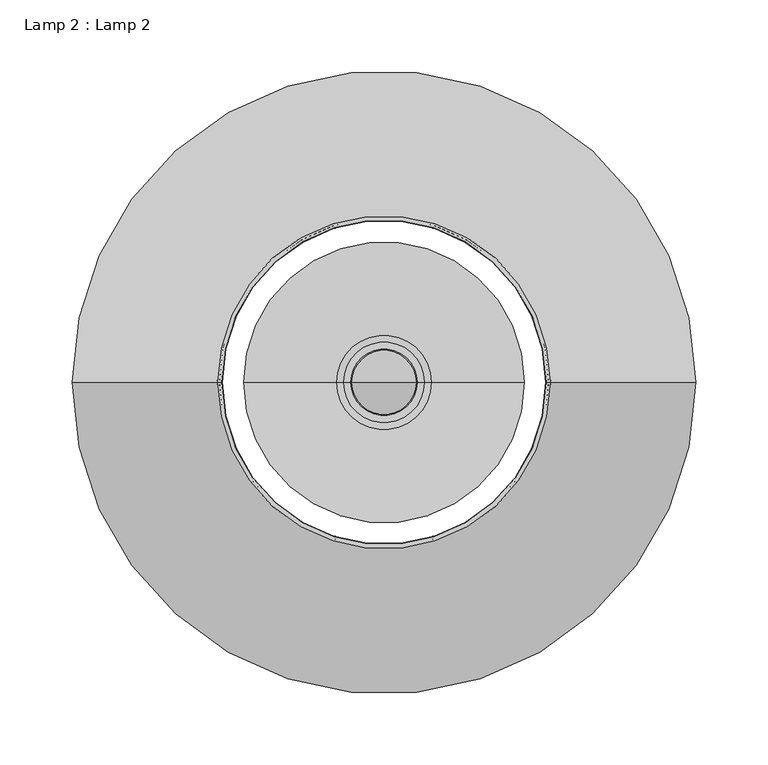
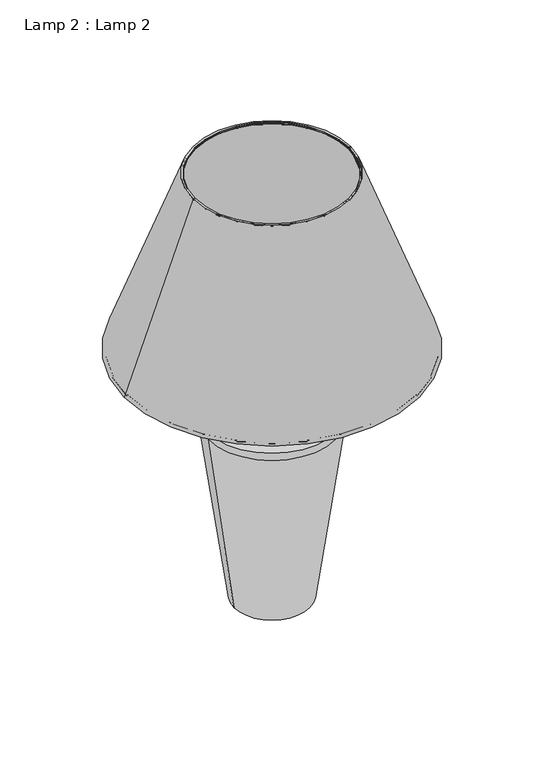
"""IFC4 building model written with IfcOpenShell, lengths in millimetres: furniture geometry, Lamp 2 : Lamp 2."""

import ifcopenshell
import ifcopenshell.guid

model = None  # the IFC model being written
_history = None  # IfcOwnerHistory: only IFC2X3 demands one
_inside = {}  # id of a spatial element -> (the spatial element, [elements in it])
_under = {}  # id of a project, library or spatial element -> (it, [spatial elements below it])
_declared = {}  # id of a project -> (the project, [libraries it declares])
_typed = {}  # id of a type object -> (the type object, [elements of that type])
_made_of = {}  # id of a material, layer set ... -> (it, [elements and type objects made of it])


def new_model(schema):
    """Start an empty IFC model of exactly this schema.

    Asked for "IFC4X3", IfcOpenShell would pick the latest addendum, in which some entities
    have other attributes; the version numbers below select the first issue.
    IFC2X3 requires an IfcOwnerHistory on every rooted entity: one is made here for all.
    """
    global model, _history
    if schema == "IFC4X3":
        model = ifcopenshell.file(schema_version=(4, 3, 0, 0))
    else:
        model = ifcopenshell.file(schema=schema)
    _inside.clear()
    _under.clear()
    _declared.clear()
    _typed.clear()
    _made_of.clear()
    _history = None
    if model.schema == "IFC2X3":
        org = make("IfcOrganization", Name="unknown")
        user = make(
            "IfcPersonAndOrganization",
            ThePerson=make("IfcPerson", FamilyName="unknown"),
            TheOrganization=org,
        )
        app = make(
            "IfcApplication",
            ApplicationDeveloper=org,
            Version="unknown",
            ApplicationFullName="unknown",
            ApplicationIdentifier="unknown",
        )
        _history = make(
            "IfcOwnerHistory",
            OwningUser=user,
            OwningApplication=app,
            ChangeAction="ADDED",
            CreationDate=0,
        )
    return model


def make(cls, **values):
    """One entity of the class cls with the attributes given. An attribute that is None is left unset."""
    return model.create_entity(
        cls, **{name: value for name, value in values.items() if value is not None}
    )


def rooted(cls, **values):
    """An entity with a GlobalId (a new one), such as an element, a storey or a relation."""
    return make(cls, GlobalId=ifcopenshell.guid.new(), OwnerHistory=_history, **values)


def si_unit(unit_type, name, prefix=None):
    """IfcSIUnit, for example si_unit("LENGTHUNIT", "METRE", prefix="MILLI")."""
    return make("IfcSIUnit", UnitType=unit_type, Prefix=prefix, Name=name)


def assignment(units):
    """IfcUnitAssignment: the units of a project."""
    return None if units is None else make("IfcUnitAssignment", Units=units)


def point(xyz):
    """IfcCartesianPoint."""
    return None if xyz is None else make("IfcCartesianPoint", Coordinates=xyz)


def direction(xyz):
    """IfcDirection."""
    return None if xyz is None else make("IfcDirection", DirectionRatios=xyz)


def frame(location, z_axis=None, x_axis=None):
    """IfcAxis2Placement3D, a coordinate frame: its origin and axes. An axis left out is left unset."""
    return make(
        "IfcAxis2Placement3D",
        Location=point(location),
        Axis=direction(z_axis),
        RefDirection=direction(x_axis),
    )


def origin():
    """The frame at (0, 0, 0) with its axes left unset."""
    return frame((0.0, 0.0, 0.0))


def place(relative_to, where):
    """IfcLocalPlacement: puts the frame where relative to a parent placement (None: the world)."""
    return make(
        "IfcLocalPlacement", PlacementRelTo=relative_to, RelativePlacement=where
    )


def context(
    kind, dimensions, precision=None, world=None, true_north=None, identifier=None
):
    """IfcGeometricRepresentationContext, for example the 3D "Model" context."""
    return make(
        "IfcGeometricRepresentationContext",
        ContextIdentifier=identifier,
        ContextType=kind,
        CoordinateSpaceDimension=dimensions,
        Precision=precision,
        WorldCoordinateSystem=world,
        TrueNorth=true_north,
    )


def project(units=None, contexts=None):
    """IfcProject with its units and contexts."""
    return rooted(
        "IfcProject",
        Name="project",
        RepresentationContexts=contexts,
        UnitsInContext=assignment(units),
    )


def spatial(cls, under=None, at=None, **own):
    """A site, building, storey or space (cls), placed at a placement, below another one or the project."""
    s = rooted(cls, ObjectPlacement=at, **own)
    if under is not None:
        _under.setdefault(under.id(), (under, []))[1].append(s)
    return s


def polyline(points):
    """IfcPolyline through the points."""
    return make("IfcPolyline", Points=[point(p) for p in points])


def circle_curve(where, radius):
    """IfcCircle in the frame where."""
    return make("IfcCircle", Position=where, Radius=radius)


def ellipse_curve(where, semi_axis1, semi_axis2):
    """IfcEllipse in the frame where."""
    return make(
        "IfcEllipse", Position=where, SemiAxis1=semi_axis1, SemiAxis2=semi_axis2
    )


def trimmed(basis, trim1, trim2, sense, master):
    """IfcTrimmedCurve: the piece of a basis curve between two trims."""
    return make(
        "IfcTrimmedCurve",
        BasisCurve=basis,
        Trim1=trim1,
        Trim2=trim2,
        SenseAgreement=sense,
        MasterRepresentation=master,
    )


def shape(context_of_items, identifier, shape_type, items):
    """IfcShapeRepresentation: the items that make up one representation, for example the "Body"."""
    return make(
        "IfcShapeRepresentation",
        ContextOfItems=context_of_items,
        RepresentationIdentifier=identifier,
        RepresentationType=shape_type,
        Items=items,
    )


def source(mapping_origin, context_of_items, identifier, shape_type, items):
    """IfcRepresentationMap: a shape defined once, which mapped items show again and again."""
    return make(
        "IfcRepresentationMap",
        MappingOrigin=mapping_origin,
        MappedRepresentation=shape(context_of_items, identifier, shape_type, items),
    )


def transform(
    local_origin,
    x_axis=None,
    y_axis=None,
    z_axis=None,
    scale=None,
    scale2=None,
    scale3=None,
    uniform=True,
):
    """IfcCartesianTransformationOperator3D, or its non-uniform kind. x_axis, y_axis, z_axis: its Axis1, 2, 3."""
    if uniform:
        return make(
            "IfcCartesianTransformationOperator3D",
            Axis1=direction(x_axis),
            Axis2=direction(y_axis),
            LocalOrigin=point(local_origin),
            Scale=scale,
            Axis3=direction(z_axis),
        )
    return make(
        "IfcCartesianTransformationOperator3DnonUniform",
        Axis1=direction(x_axis),
        Axis2=direction(y_axis),
        LocalOrigin=point(local_origin),
        Scale=scale,
        Axis3=direction(z_axis),
        Scale2=scale2,
        Scale3=scale3,
    )


def mapped(mapping_source, mapping_target):
    """IfcMappedItem: shows the shape of a source again, moved by a transform."""
    return make(
        "IfcMappedItem", MappingSource=mapping_source, MappingTarget=mapping_target
    )


def made_of(thing, what):
    """Note that an element or type object is made of a material, layer set ...; save() writes the relation."""
    if what is not None:
        _made_of.setdefault(what.id(), (what, []))[1].append(thing)
    return thing


def element(
    cls,
    number,
    at=None,
    inside=None,
    cuts=None,
    type_object=None,
    material=None,
    context=None,
    identifier="Body",
    shape_type=None,
    held_by="IfcProductDefinitionShape",
    body=None,
    shapes=None,
    **own,
):
    """One element of the class cls, such as IfcWall. Its Tag is "e" and its number.

    at: its placement. inside: the storey or other place that contains it. cuts: it is an
    opening in that element (IfcRelVoidsElement). A single representation is given by context,
    identifier, shape_type and body (its items); several are given by shapes. held_by: the class
    of the entity that holds the representations. save() writes the other relations.
    """
    e = rooted(cls, Tag="e%d" % number, ObjectPlacement=at, **own)
    if body is not None:
        shapes = [shape(context, identifier, shape_type, body)]
    if shapes is not None:
        e.Representation = make(held_by, Representations=shapes)
    if inside is not None:
        _inside.setdefault(inside.id(), (inside, []))[1].append(e)
    if cuts is not None:
        rooted(
            "IfcRelVoidsElement", RelatingBuildingElement=cuts, RelatedOpeningElement=e
        )
    if type_object is not None:
        _typed.setdefault(type_object.id(), (type_object, []))[1].append(e)
    return made_of(e, material)


def aggregate(whole, parts):
    """IfcRelAggregates: a whole, such as a stair, and the parts it consists of."""
    return rooted("IfcRelAggregates", RelatingObject=whole, RelatedObjects=parts)


def save(model, path):
    """Write the relations noted so far, then the file.

    IfcRelAggregates (storeys below a building ...), IfcRelContainedInSpatialStructure (elements
    in a storey), IfcRelDefinesByType, IfcRelAssociatesMaterial and IfcRelDeclares: one each for
    every whole, place, type object, material and project.
    """
    for whole, parts in _under.values():
        aggregate(whole, parts)
    for where, things in _inside.values():
        rooted(
            "IfcRelContainedInSpatialStructure",
            RelatedElements=things,
            RelatingStructure=where,
        )
    for kind, things in _typed.values():
        rooted("IfcRelDefinesByType", RelatedObjects=things, RelatingType=kind)
    for what, things in _made_of.values():
        rooted("IfcRelAssociatesMaterial", RelatedObjects=things, RelatingMaterial=what)
    for by, libraries in _declared.values():
        rooted("IfcRelDeclares", RelatingContext=by, RelatedDefinitions=libraries)
    model.write(path)


def plane_surface(at):
    """IfcPlane: the flat surface through the origin of the frame at, square to its z axis."""
    return make("IfcPlane", Position=at)


def cylinder_surface(at, radius):
    """IfcCylindricalSurface: all points at the distance radius from the z axis of the frame at."""
    return make("IfcCylindricalSurface", Position=at, Radius=radius)


def revolved_surface(curve, axis_point, axis_direction):
    """IfcSurfaceOfRevolution: the curve turned about the line through axis_point along axis_direction."""
    return make(
        "IfcSurfaceOfRevolution",
        SweptCurve=make("IfcArbitraryOpenProfileDef", ProfileType="CURVE", Curve=curve),
        AxisPosition=make("IfcAxis1Placement", Location=point(axis_point), Axis=direction(axis_direction)),
    )


def spline_curve(degree, points, multiplicities, knots, weights=None):
    """IfcBSplineCurveWithKnots; with weights, IfcRationalBSplineCurveWithKnots."""
    own = dict(
        Degree=degree,
        ControlPointsList=[point(p) for p in points],
        CurveForm="UNSPECIFIED",
        ClosedCurve=False,
        SelfIntersect=False,
        KnotMultiplicities=multiplicities,
        Knots=knots,
        KnotSpec="UNSPECIFIED",
    )
    if weights is None:
        return make("IfcBSplineCurveWithKnots", **own)
    return make("IfcRationalBSplineCurveWithKnots", WeightsData=weights, **own)


def advanced_brep(points, edges, surfaces, faces):
    """IfcAdvancedBrep: a solid bounded by faces that lie on surfaces and meet in shared edges.

    An edge is (start, end): straight between two places in points (the first is 0);
    or (start, end, curve); or (start, end, curve, False) where it runs against its curve.
    A face is (place in surfaces, loops), or (place, loops, False) where it looks against
    its surface's normal. A loop lists edges by number (the first is 1), with a minus sign
    where the edge is run from its end to its start. The first loop is the outer one.
    """
    corners = [point(p) for p in points]
    vertices = [make("IfcVertexPoint", VertexGeometry=c) for c in corners]
    made = []
    for start, end, *more in edges:
        made.append(
            make(
                "IfcEdgeCurve",
                EdgeStart=vertices[start],
                EdgeEnd=vertices[end],
                EdgeGeometry=more[0] if more else make("IfcPolyline", Points=[corners[start], corners[end]]),
                SameSense=more[1] if len(more) > 1 else True,
            )
        )
    hull = []
    for where, loops, *sense in faces:
        bounds = []
        for j, loop in enumerate(loops):
            ring = [make("IfcOrientedEdge", EdgeElement=made[abs(k) - 1], Orientation=k > 0) for k in loop]
            bounds.append(
                make(
                    "IfcFaceOuterBound" if j == 0 else "IfcFaceBound",
                    Bound=make("IfcEdgeLoop", EdgeList=ring),
                    Orientation=True,
                )
            )
        hull.append(make("IfcAdvancedFace", Bounds=bounds, FaceSurface=surfaces[where], SameSense=sense[0] if sense else True))
    return make("IfcAdvancedBrep", Outer=make("IfcClosedShell", CfsFaces=hull))


def lamp_2_lamp_2_ee5345a8(model_context):
    return source(origin(), model_context, "Body", "AdvancedBrep", [
        advanced_brep(
        [(-5.625, 0.0049096, 408.6874636), (5.625, 0.0049096, 408.6874636), (5.625, 0.0049096, 396.7479044), (-5.625, 0.0049096, 396.7479044), (0.0, 0.0049096, 452.3091199), (0.0, 0.0049096, 396.7479044)],
        [
            (0, 1, circle_curve(frame((0.0, 0.0049096, 408.6874636), z_axis=(0.0, 0.0, -1.0), x_axis=(1.0, 0.0, 0.0)), 5.625)),
            (1, 2),
            (2, 3, circle_curve(frame((0.0, 0.0049096, 396.7479044), z_axis=(0.0, 0.0, 1.0), x_axis=(1.0, 0.0, 0.0)), 5.625)),
            (3, 0),
            (1, 0, circle_curve(frame((0.0, 0.0049096, 408.6874636), z_axis=(0.0, 0.0, -1.0), x_axis=(1.0, 0.0, 0.0)), 5.625)),
            (3, 2, circle_curve(frame((0.0, 0.0049096, 396.7479044), z_axis=(0.0, 0.0, 1.0), x_axis=(1.0, 0.0, 0.0)), 5.625)),
            (4, 1, circle_curve(frame((0.0, 0.0049096, 430.1356207), z_axis=(0.0, 1.0, 0.0), x_axis=(1.0, 0.0, 0.0)), 22.1734992)),
            (0, 4, circle_curve(frame((0.0, 0.0049096, 430.1356207), z_axis=(0.0, 1.0, 0.0), x_axis=(-1.0, 0.0, 0.0)), 22.1734992)),
            (2, 5),
            (5, 3),
        ],
        [
            cylinder_surface(frame((0.0, 0.0049096, 452.3091199), z_axis=(0.0, 0.0, 1.0), x_axis=(1.0, 0.0, 0.0)), 5.625),
            revolved_surface(trimmed(ellipse_curve(frame((0.0, 0.0049096, 430.1356207), z_axis=(0.0, -1.0, 0.0), x_axis=(1.0, 0.0, 0.0)), 22.1734992, 22.1734992), [point((5.625, 0.0049096, 408.6874636))], [point((0.0, 0.0049096, 452.3091199))], True, "CARTESIAN"), (0.0, 0.0049096, 452.3091199), (0.0, 0.0, 1.0)),
            plane_surface(frame((0.0, 0.0049096, 396.7479044), z_axis=(0.0, 0.0, -1.0), x_axis=(1.0, 0.0, 0.0))),
        ],
        [
            (0, [[1, 2, 3, 4]]),
            (0, [[5, -4, 6, -2]]),
            (1, [[7, -1, 8]]),
            (1, [[-8, -5, -7]]),
            (2, [[-3, 9, 10]]),
            (2, [[-6, -10, -9]]),
        ],
    ),
        advanced_brep(
        [(210.2699359, 0.0, 381.7682447), (-210.1136859, 0.0, 381.7682447), (-212.1136859, 0.0, 381.7682447), (212.2699359, 0.0, 381.7682447)],
        [
            (0, 1, circle_curve(frame((0.078125, 0.0, 381.7682447), z_axis=(0.0, 0.0, 1.0), x_axis=(-1.0, 0.0, 0.0)), 210.1918109)),
            (1, 2, circle_curve(frame((-211.1136859, 0.0, 381.7682447), z_axis=(0.0, 1.0, 0.0), x_axis=(1.0, 0.0, 0.0)), 1.0)),
            (2, 3, circle_curve(frame((0.078125, 0.0, 381.7682447), z_axis=(0.0, 0.0, -1.0), x_axis=(-1.0, 0.0, 0.0)), 212.1918109)),
            (3, 0, circle_curve(frame((211.2699359, 0.0, 381.7682447), z_axis=(0.0, 1.0, 0.0), x_axis=(-1.0, 0.0, 0.0)), 1.0)),
            (1, 0, circle_curve(frame((0.078125, 0.0, 381.7682447), z_axis=(0.0, 0.0, 1.0), x_axis=(-1.0, 0.0, 0.0)), 210.1918109)),
            (3, 2, circle_curve(frame((0.078125, 0.0, 381.7682447), z_axis=(0.0, 0.0, -1.0), x_axis=(-1.0, 0.0, 0.0)), 212.1918109)),
            (2, 1, circle_curve(frame((-211.1136859, 0.0, 381.7682447), z_axis=(0.0, 1.0, 0.0), x_axis=(1.0, 0.0, 0.0)), 1.0)),
            (0, 3, circle_curve(frame((211.2699359, 0.0, 381.7682447), z_axis=(0.0, 1.0, 0.0), x_axis=(-1.0, 0.0, 0.0)), 1.0)),
        ],
        [
            revolved_surface(trimmed(ellipse_curve(frame((-211.1136859, 0.0, 381.7682447), z_axis=(0.0, -1.0, 0.0), x_axis=(1.0, 0.0, 0.0)), 1.0, 1.0), [point((-212.1136859, 0.0, 381.7682447))], [point((-210.1136859, 0.0, 381.7682447))], True, "CARTESIAN"), (0.078125, 0.0, 370.9862512), (0.0, 0.0, -1.0)),
            revolved_surface(trimmed(ellipse_curve(frame((-211.1136859, 0.0, 381.7682447), z_axis=(0.0, -1.0, 0.0), x_axis=(1.0, 0.0, 0.0)), 1.0, 1.0), [point((-210.1136859, 0.0, 381.7682447))], [point((-212.1136859, 0.0, 381.7682447))], True, "CARTESIAN"), (0.078125, 0.0, 370.9862512), (0.0, 0.0, -1.0)),
        ],
        [
            (0, [[1, 2, 3, 4]]),
            (0, [[5, -4, 6, -2]]),
            (1, [[-3, 7, -1, 8]]),
            (1, [[-6, -8, -5, -7]]),
        ],
    ),
        advanced_brep(
        [(111.7827914, 0.0, 647.8021308), (-111.7827914, 0.0, 647.8021308), (-113.7827914, 0.0, 647.8021308), (113.7827914, 0.0, 647.8021308)],
        [
            (0, 1, circle_curve(frame((0.0, 0.0, 647.8021308), z_axis=(0.0, 0.0, 1.0), x_axis=(-1.0, 0.0, 0.0)), 111.7827914)),
            (1, 2, circle_curve(frame((-112.7827914, 0.0, 647.8021308), z_axis=(0.0, 1.0, 0.0), x_axis=(1.0, 0.0, 0.0)), 1.0)),
            (2, 3, circle_curve(frame((0.0, 0.0, 647.8021308), z_axis=(0.0, 0.0, -1.0), x_axis=(-1.0, 0.0, 0.0)), 113.7827914)),
            (3, 0, circle_curve(frame((112.7827914, 0.0, 647.8021308), z_axis=(0.0, 1.0, 0.0), x_axis=(-1.0, 0.0, 0.0)), 1.0)),
            (1, 0, circle_curve(frame((0.0, 0.0, 647.8021308), z_axis=(0.0, 0.0, 1.0), x_axis=(-1.0, 0.0, 0.0)), 111.7827914)),
            (3, 2, circle_curve(frame((0.0, 0.0, 647.8021308), z_axis=(0.0, 0.0, -1.0), x_axis=(-1.0, 0.0, 0.0)), 113.7827914)),
            (2, 1, circle_curve(frame((-112.7827914, 0.0, 647.8021308), z_axis=(0.0, 1.0, 0.0), x_axis=(1.0, 0.0, 0.0)), 1.0)),
            (0, 3, circle_curve(frame((112.7827914, 0.0, 647.8021308), z_axis=(0.0, 1.0, 0.0), x_axis=(-1.0, 0.0, 0.0)), 1.0)),
        ],
        [
            revolved_surface(trimmed(ellipse_curve(frame((-112.7827914, 0.0, 647.8021308), z_axis=(0.0, -1.0, 0.0), x_axis=(1.0, 0.0, 0.0)), 1.0, 1.0), [point((-113.7827914, 0.0, 647.8021308))], [point((-111.7827914, 0.0, 647.8021308))], True, "CARTESIAN"), (0.0, 0.0, 669.21875), (0.0, 0.0, -1.0)),
            revolved_surface(trimmed(ellipse_curve(frame((-112.7827914, 0.0, 647.8021308), z_axis=(0.0, -1.0, 0.0), x_axis=(1.0, 0.0, 0.0)), 1.0, 1.0), [point((-111.7827914, 0.0, 647.8021308))], [point((-113.7827914, 0.0, 647.8021308))], True, "CARTESIAN"), (0.0, 0.0, 669.21875), (0.0, 0.0, -1.0)),
        ],
        [
            (0, [[1, 2, 3, 4]]),
            (0, [[5, -4, 6, -2]]),
            (1, [[-3, 7, -1, 8]]),
            (1, [[-6, -8, -5, -7]]),
        ],
    ),
        advanced_brep(
        [(0.0, 0.0, 380.0), (-32.5, 0.0, 380.0), (32.5, 0.0, 380.0), (10.0478847, 0.0, 406.8452028), (-10.0478847, 0.0, 406.8452028), (0.0, 0.0, 406.8452028), (7.1801044, 0.0, 396.1425012), (-7.1801044, 0.0, 396.1425012), (8.4301044, 0.0, 396.1425012), (-8.4301044, 0.0, 396.1425012), (13.1200696, 0.0, 393.7368661), (-13.1200696, 0.0, 393.7368661), (13.1200696, 0.0, 390.7616675), (-13.1200696, 0.0, 390.7616675), (18.1200696, 0.0, 390.7616675), (-18.1200696, 0.0, 390.7616675), (22.8100348, 0.0, 388.3560323), (-22.8100348, 0.0, 388.3560323), (22.8100348, 0.0, 385.3808337), (-22.8100348, 0.0, 385.3808337), (27.8100348, 0.0, 385.3808337), (-27.8100348, 0.0, 385.3808337), (32.5, 0.0, 382.9751986), (-32.5, 0.0, 382.9751986)],
        [
            (0, 1),
            (1, 2, circle_curve(frame((0.0, 0.0, 380.0), z_axis=(0.0, 0.0, -1.0), x_axis=(-1.0, 0.0, 0.0)), 32.5)),
            (2, 0),
            (2, 1, circle_curve(frame((0.0, 0.0, 380.0), z_axis=(0.0, 0.0, -1.0), x_axis=(-1.0, 0.0, 0.0)), 32.5)),
            (3, 4, circle_curve(frame((0.0, 0.0, 406.8452028), z_axis=(0.0, 0.0, 1.0), x_axis=(-1.0, 0.0, 0.0)), 10.0478847)),
            (4, 5),
            (5, 3),
            (4, 3, circle_curve(frame((0.0, 0.0, 406.8452028), z_axis=(0.0, 0.0, 1.0), x_axis=(-1.0, 0.0, 0.0)), 10.0478847)),
            (6, 7, circle_curve(frame((0.0, 0.0, 396.1425012), z_axis=(0.0, 0.0, 1.0), x_axis=(-1.0, 0.0, 0.0)), 7.1801044)),
            (7, 4),
            (3, 6),
            (7, 6, circle_curve(frame((0.0, 0.0, 396.1425012), z_axis=(0.0, 0.0, 1.0), x_axis=(-1.0, 0.0, 0.0)), 7.1801044)),
            (8, 9, circle_curve(frame((0.0, 0.0, 396.1425012), z_axis=(0.0, 0.0, 1.0), x_axis=(-1.0, 0.0, 0.0)), 8.4301044)),
            (9, 7),
            (6, 8),
            (9, 8, circle_curve(frame((0.0, 0.0, 396.1425012), z_axis=(0.0, 0.0, 1.0), x_axis=(-1.0, 0.0, 0.0)), 8.4301044)),
            (10, 11, circle_curve(frame((0.0, 0.0, 393.7368661), z_axis=(0.0, 0.0, 1.0), x_axis=(-1.0, 0.0, 0.0)), 13.1200696)),
            (11, 9, circle_curve(frame((-7.7356139, 0.0, 389.0140039), z_axis=(0.0, 1.0, 0.0), x_axis=(1.0, 0.0, 0.0)), 7.1622476)),
            (8, 10, circle_curve(frame((7.7356139, 0.0, 389.0140039), z_axis=(0.0, 1.0, 0.0), x_axis=(-1.0, 0.0, 0.0)), 7.1622476)),
            (11, 10, circle_curve(frame((0.0, 0.0, 393.7368661), z_axis=(0.0, 0.0, 1.0), x_axis=(-1.0, 0.0, 0.0)), 13.1200696)),
            (12, 13, circle_curve(frame((0.0, 0.0, 390.7616675), z_axis=(0.0, 0.0, 1.0), x_axis=(-1.0, 0.0, 0.0)), 13.1200696)),
            (13, 11),
            (10, 12),
            (13, 12, circle_curve(frame((0.0, 0.0, 390.7616675), z_axis=(0.0, 0.0, 1.0), x_axis=(-1.0, 0.0, 0.0)), 13.1200696)),
            (14, 15, circle_curve(frame((0.0, 0.0, 390.7616675), z_axis=(0.0, 0.0, 1.0), x_axis=(-1.0, 0.0, 0.0)), 18.1200696)),
            (15, 13),
            (12, 14),
            (15, 14, circle_curve(frame((0.0, 0.0, 390.7616675), z_axis=(0.0, 0.0, 1.0), x_axis=(-1.0, 0.0, 0.0)), 18.1200696)),
            (16, 17, circle_curve(frame((0.0, 0.0, 388.3560323), z_axis=(0.0, 0.0, 1.0), x_axis=(-1.0, 0.0, 0.0)), 22.8100348)),
            (17, 15, circle_curve(frame((-17.4255791, 0.0, 383.6331702), z_axis=(0.0, 1.0, 0.0), x_axis=(1.0, 0.0, 0.0)), 7.1622476)),
            (14, 16, circle_curve(frame((17.4255791, 0.0, 383.6331702), z_axis=(0.0, 1.0, 0.0), x_axis=(-1.0, 0.0, 0.0)), 7.1622476)),
            (17, 16, circle_curve(frame((0.0, 0.0, 388.3560323), z_axis=(0.0, 0.0, 1.0), x_axis=(-1.0, 0.0, 0.0)), 22.8100348)),
            (18, 19, circle_curve(frame((0.0, 0.0, 385.3808337), z_axis=(0.0, 0.0, 1.0), x_axis=(-1.0, 0.0, 0.0)), 22.8100348)),
            (19, 17),
            (16, 18),
            (19, 18, circle_curve(frame((0.0, 0.0, 385.3808337), z_axis=(0.0, 0.0, 1.0), x_axis=(-1.0, 0.0, 0.0)), 22.8100348)),
            (20, 21, circle_curve(frame((0.0, 0.0, 385.3808337), z_axis=(0.0, 0.0, 1.0), x_axis=(-1.0, 0.0, 0.0)), 27.8100348)),
            (21, 19),
            (18, 20),
            (21, 20, circle_curve(frame((0.0, 0.0, 385.3808337), z_axis=(0.0, 0.0, 1.0), x_axis=(-1.0, 0.0, 0.0)), 27.8100348)),
            (22, 23, circle_curve(frame((0.0, 0.0, 382.9751986), z_axis=(0.0, 0.0, 1.0), x_axis=(-1.0, 0.0, 0.0)), 32.5)),
            (23, 21, circle_curve(frame((-27.1155443, 0.0, 378.2523365), z_axis=(0.0, 1.0, 0.0), x_axis=(1.0, 0.0, 0.0)), 7.1622476)),
            (20, 22, circle_curve(frame((27.1155443, 0.0, 378.2523365), z_axis=(0.0, 1.0, 0.0), x_axis=(-1.0, 0.0, 0.0)), 7.1622476)),
            (23, 22, circle_curve(frame((0.0, 0.0, 382.9751986), z_axis=(0.0, 0.0, 1.0), x_axis=(-1.0, 0.0, 0.0)), 32.5)),
            (1, 23),
            (22, 2),
        ],
        [
            plane_surface(frame((0.0, 0.0, 380.0), z_axis=(0.0, 0.0, -1.0), x_axis=(-1.0, 0.0, 0.0))),
            plane_surface(frame((0.0, 0.0, 406.8452028), z_axis=(0.0, 0.0, 1.0), x_axis=(-1.0, 0.0, 0.0))),
            revolved_surface(polyline([(-10.0478847, 0.0, 406.8452028), (-7.1801044, 0.0, 396.1425012)]), (0.0, 0.0, 417.9746199), (0.0, 0.0, -1.0)),
            plane_surface(frame((0.0, 0.0, 396.1425012), z_axis=(0.0, 0.0, 1.0), x_axis=(-1.0, 0.0, 0.0))),
            revolved_surface(trimmed(ellipse_curve(frame((-7.7356139, 0.0, 389.0140039), z_axis=(0.0, -1.0, 0.0), x_axis=(1.0, 0.0, 0.0)), 7.1622476, 7.1622476), [point((-8.4301044, 0.0, 396.1425012))], [point((-13.1200696, 0.0, 393.7368661))], True, "CARTESIAN"), (0.0, 0.0, 417.9746199), (0.0, 0.0, -1.0)),
            cylinder_surface(frame((0.0, 0.0, 417.9746199), z_axis=(0.0, 0.0, -1.0), x_axis=(-1.0, 0.0, 0.0)), 13.1200696),
            plane_surface(frame((0.0, 0.0, 390.7616675), z_axis=(0.0, 0.0, 1.0), x_axis=(-1.0, 0.0, 0.0))),
            revolved_surface(trimmed(ellipse_curve(frame((-17.4255791, 0.0, 383.6331702), z_axis=(0.0, -1.0, 0.0), x_axis=(1.0, 0.0, 0.0)), 7.1622476, 7.1622476), [point((-18.1200696, 0.0, 390.7616675))], [point((-22.8100348, 0.0, 388.3560323))], True, "CARTESIAN"), (0.0, 0.0, 417.9746199), (0.0, 0.0, -1.0)),
            cylinder_surface(frame((0.0, 0.0, 417.9746199), z_axis=(0.0, 0.0, -1.0), x_axis=(-1.0, 0.0, 0.0)), 22.8100348),
            plane_surface(frame((0.0, 0.0, 385.3808337), z_axis=(0.0, 0.0, 1.0), x_axis=(-1.0, 0.0, 0.0))),
            revolved_surface(trimmed(ellipse_curve(frame((-27.1155443, 0.0, 378.2523365), z_axis=(0.0, -1.0, 0.0), x_axis=(1.0, 0.0, 0.0)), 7.1622476, 7.1622476), [point((-27.8100348, 0.0, 385.3808337))], [point((-32.5, 0.0, 382.9751986))], True, "CARTESIAN"), (0.0, 0.0, 417.9746199), (0.0, 0.0, -1.0)),
            cylinder_surface(frame((0.0, 0.0, 417.9746199), z_axis=(0.0, 0.0, -1.0), x_axis=(-1.0, 0.0, 0.0)), 32.5),
        ],
        [
            (0, [[1, 2, 3]]),
            (0, [[-3, 4, -1]]),
            (1, [[5, 6, 7]]),
            (1, [[8, -7, -6]]),
            (2, [[9, 10, -5, 11]]),
            (2, [[12, -11, -8, -10]]),
            (3, [[13, 14, -9, 15]]),
            (3, [[16, -15, -12, -14]]),
            (4, [[17, 18, -13, 19]]),
            (4, [[20, -19, -16, -18]]),
            (5, [[21, 22, -17, 23]]),
            (5, [[24, -23, -20, -22]]),
            (6, [[25, 26, -21, 27]]),
            (6, [[28, -27, -24, -26]]),
            (7, [[29, 30, -25, 31]]),
            (7, [[32, -31, -28, -30]]),
            (8, [[33, 34, -29, 35]]),
            (8, [[36, -35, -32, -34]]),
            (9, [[37, 38, -33, 39]]),
            (9, [[40, -39, -36, -38]]),
            (10, [[41, 42, -37, 43]]),
            (10, [[44, -43, -40, -42]]),
            (11, [[-2, 45, -41, 46]]),
            (11, [[-4, -46, -44, -45]]),
        ],
    ),
        advanced_brep(
        [(55.0, 0.0, 0.0), (-55.0, 0.0, 0.0), (-93.2726028, 0.0, 272.3237189), (93.2726028, 0.0, 272.3237189), (0.0, 0.0, 0.0), (32.5, 0.0, 380.0), (-32.5, 0.0, 380.0), (0.0, 0.0, 380.0), (95.0446085, 0.0, 284.932195), (-95.0446085, 0.0, 284.932195)],
        [
            (0, 1, circle_curve(frame((0.0, 0.0, 0.0), z_axis=(0.0, 0.0, 1.0), x_axis=(-1.0, 0.0, 0.0)), 55.0)),
            (1, 2),
            (2, 3, circle_curve(frame((0.0, 0.0, 272.3237189), z_axis=(0.0, 0.0, -1.0), x_axis=(-1.0, 0.0, 0.0)), 93.2726028)),
            (3, 0),
            (1, 0, circle_curve(frame((0.0, 0.0, 0.0), z_axis=(0.0, 0.0, 1.0), x_axis=(-1.0, 0.0, 0.0)), 55.0)),
            (3, 2, circle_curve(frame((0.0, 0.0, 272.3237189), z_axis=(0.0, 0.0, -1.0), x_axis=(-1.0, 0.0, 0.0)), 93.2726028)),
            (4, 1),
            (0, 4),
            (5, 6, circle_curve(frame((0.0, 0.0, 380.0), z_axis=(0.0, 0.0, 1.0), x_axis=(-1.0, 0.0, 0.0)), 32.5)),
            (6, 7),
            (7, 5),
            (6, 5, circle_curve(frame((0.0, 0.0, 380.0), z_axis=(0.0, 0.0, 1.0), x_axis=(-1.0, 0.0, 0.0)), 32.5)),
            (8, 9, circle_curve(frame((0.0, 0.0, 284.932195), z_axis=(0.0, 0.0, 1.0), x_axis=(-1.0, 0.0, 0.0)), 95.0446085)),
            (9, 6, spline_curve(3, [(-95.0446085, 0.0, 284.932195), (-97.453949935, 0.0, 298.596249282), (-96.188694178, 0.0, 303.810562504), (-91.4761635, 0.0, 311.111813345), (-87.982441251, 0.0, 313.128914852), (-80.007669597, 0.0, 317.691178928), (-75.616399887, 0.0, 320.187545578), (-71.996617923, 0.0, 325.651073111), (-71.996617881, 0.0, 328.458469354), (-71.615996393, 0.0, 332.724687482), (-71.353175804, 0.0, 334.331973474), (-70.786475665, 0.0, 337.797642111), (-70.481715894, 0.0, 339.661407947), (-71.254006942, 0.0, 343.624329421), (-72.504543085, 0.0, 345.724406697), (-76.143249721, 0.0, 350.099491704), (-78.742373361, 0.0, 351.600096459), (-86.562175204, 0.0, 356.114861157), (-92.020074445, 0.0, 359.265980803), (-98.470606982, 0.0, 366.885189171), (-97.195457616, 0.0, 371.424256987), (-88.6243529, 0.0, 376.130489061), (-81.983535995, 0.0, 376.711485228), (-67.143390223, 0.0, 378.570660036), (-59.037200537, 0.0, 380.0), (-32.5, 0.0, 380.0)], [4, 2, 2, 2, 2, 2, 2, 2, 2, 2, 2, 2, 4], [0.0, 0.03985914919293754, 0.08057749635778949, 0.11834827401611286, 0.14948322781927886, 0.17098203520545735, 0.19303228957060214, 0.21777825276599289, 0.2586170795711167, 0.30356033835425955, 0.3644303221319498, 0.4188228813927918, 0.48866624030450706])),
            (5, 8, spline_curve(3, [(32.5, 0.0, 380.0), (59.037200537, 0.0, 380.0), (67.143390223, 0.0, 378.570660036), (81.983535995, 0.0, 376.711485228), (88.6243529, 0.0, 376.130489061), (97.195457616, 0.0, 371.424256987), (98.470606982, 0.0, 366.885189171), (92.020074445, 0.0, 359.265980803), (86.562175204, 0.0, 356.114861157), (78.742373361, 0.0, 351.600096459), (76.143249721, 0.0, 350.099491704), (72.504543085, 0.0, 345.724406697), (71.254006942, 0.0, 343.624329421), (70.481715894, 0.0, 339.661407947), (70.786475665, 0.0, 337.797642111), (71.353175804, 0.0, 334.331973474), (71.615996393, 0.0, 332.724687482), (71.996617881, 0.0, 328.458469354), (71.996617923, 0.0, 325.651073111), (75.616399887, 0.0, 320.187545578), (80.007669597, 0.0, 317.691178928), (87.982441251, 0.0, 313.128914852), (91.4761635, 0.0, 311.111813345), (96.188694178, 0.0, 303.810562504), (97.453949935, 0.0, 298.596249282), (95.0446085, 0.0, 284.932195)], [4, 2, 2, 2, 2, 2, 2, 2, 2, 2, 2, 2, 4], [0.0, 0.06984335891171527, 0.12423591817255722, 0.1851059019502475, 0.23004916073339038, 0.2708879875385142, 0.2956339507339049, 0.3176842050990497, 0.3391830124852282, 0.3703179662883942, 0.40808874394671757, 0.4488070911115695, 0.48866624030450706])),
            (9, 8, circle_curve(frame((0.0, 0.0, 284.932195), z_axis=(0.0, 0.0, 1.0), x_axis=(-1.0, 0.0, 0.0)), 95.0446085)),
            (2, 9),
            (8, 3),
        ],
        [
            revolved_surface(polyline([(-93.2726028, 0.0, 272.3237189), (-55.0, 0.0, 0.0)]), (0.0, 0.0, 420.0), (0.0, 0.0, -1.0)),
            plane_surface(frame((0.0, 0.0, 0.0), z_axis=(0.0, 0.0, -1.0), x_axis=(-1.0, 0.0, 0.0))),
            plane_surface(frame((0.0, 0.0, 380.0), z_axis=(0.0, 0.0, 1.0), x_axis=(-1.0, 0.0, 0.0))),
            revolved_surface(spline_curve(3, [(-32.5, 0.0, 380.0), (-59.037200537, 0.0, 380.0), (-67.143390223, 0.0, 378.570660036), (-81.983535995, 0.0, 376.711485228), (-88.6243529, 0.0, 376.130489061), (-97.195457616, 0.0, 371.424256987), (-98.470606982, 0.0, 366.885189171), (-92.020074445, 0.0, 359.265980803), (-86.562175204, 0.0, 356.114861157), (-78.742373361, 0.0, 351.600096459), (-76.143249721, 0.0, 350.099491704), (-72.504543085, 0.0, 345.724406697), (-71.254006942, 0.0, 343.624329421), (-70.481715894, 0.0, 339.661407947), (-70.786475665, 0.0, 337.797642111), (-71.353175804, 0.0, 334.331973474), (-71.615996393, 0.0, 332.724687482), (-71.996617881, 0.0, 328.458469354), (-71.996617923, 0.0, 325.651073111), (-75.616399887, 0.0, 320.187545578), (-80.007669597, 0.0, 317.691178928), (-87.982441251, 0.0, 313.128914852), (-91.4761635, 0.0, 311.111813345), (-96.188694178, 0.0, 303.810562504), (-97.453949935, 0.0, 298.596249282), (-95.0446085, 0.0, 284.932195)], [4, 2, 2, 2, 2, 2, 2, 2, 2, 2, 2, 2, 4], [0.0, 0.06984335891171527, 0.12423591817255722, 0.1851059019502475, 0.23004916073339038, 0.2708879875385142, 0.2956339507339049, 0.3176842050990497, 0.3391830124852282, 0.3703179662883942, 0.40808874394671757, 0.4488070911115695, 0.48866624030450706]), (0.0, 0.0, 420.0), (0.0, 0.0, -1.0)),
            revolved_surface(polyline([(-95.0446085, 0.0, 284.932195), (-93.2726028, 0.0, 272.3237189)]), (0.0, 0.0, 420.0), (0.0, 0.0, -1.0)),
        ],
        [
            (0, [[1, 2, 3, 4]]),
            (0, [[5, -4, 6, -2]]),
            (1, [[7, -1, 8]]),
            (1, [[-8, -5, -7]]),
            (2, [[9, 10, 11]]),
            (2, [[12, -11, -10]]),
            (3, [[13, 14, -9, 15]]),
            (3, [[16, -15, -12, -14]]),
            (4, [[-3, 17, -13, 18]]),
            (4, [[-6, -18, -16, -17]]),
        ],
    ),
        advanced_brep(
        [(-115.0, 0.0, 650.0), (115.0, 0.0, 650.0), (215.0, 0.0, 380.0), (-215.0, 0.0, 380.0), (-111.9695243, 0.0, 650.0), (111.9695243, 0.0, 650.0), (-212.7058705, 0.0, 380.7941496), (212.7058705, 0.0, 380.7941496), (113.4388971, 0.0, 648.8149779), (-113.4388971, 0.0, 648.8149779), (211.2249908, 0.0, 380.0), (-211.2249908, 0.0, 380.0), (-111.9695243, 0.0, 648.8149779), (111.9695243, 0.0, 648.8149779), (-211.2249908, 0.0, 380.7941496), (211.2249908, 0.0, 380.7941496)],
        [
            (0, 1, circle_curve(frame((0.0, 0.0, 650.0), z_axis=(0.0, 0.0, -1.0), x_axis=(1.0, 0.0, 0.0)), 115.0)),
            (1, 2),
            (2, 3, circle_curve(frame((0.0, 0.0, 380.0), z_axis=(0.0, 0.0, 1.0), x_axis=(1.0, 0.0, 0.0)), 215.0)),
            (3, 0),
            (1, 0, circle_curve(frame((0.0, 0.0, 650.0), z_axis=(0.0, 0.0, -1.0), x_axis=(1.0, 0.0, 0.0)), 115.0)),
            (3, 2, circle_curve(frame((0.0, 0.0, 380.0), z_axis=(0.0, 0.0, 1.0), x_axis=(1.0, 0.0, 0.0)), 215.0)),
            (4, 5, circle_curve(frame((0.0, 0.0, 650.0), z_axis=(0.0, 0.0, -1.0), x_axis=(1.0, 0.0, 0.0)), 111.9695243)),
            (5, 1),
            (0, 4),
            (5, 4, circle_curve(frame((0.0, 0.0, 650.0), z_axis=(0.0, 0.0, -1.0), x_axis=(1.0, 0.0, 0.0)), 111.9695243)),
            (6, 7, circle_curve(frame((0.0, 0.0, 380.7941496), z_axis=(0.0, 0.0, -1.0), x_axis=(1.0, 0.0, 0.0)), 212.7058705)),
            (7, 8),
            (8, 9, circle_curve(frame((0.0, 0.0, 648.8149779), z_axis=(0.0, 0.0, 1.0), x_axis=(1.0, 0.0, 0.0)), 113.4388971)),
            (9, 6),
            (7, 6, circle_curve(frame((0.0, 0.0, 380.7941496), z_axis=(0.0, 0.0, -1.0), x_axis=(1.0, 0.0, 0.0)), 212.7058705)),
            (9, 8, circle_curve(frame((0.0, 0.0, 648.8149779), z_axis=(0.0, 0.0, 1.0), x_axis=(1.0, 0.0, 0.0)), 113.4388971)),
            (2, 10),
            (10, 11, circle_curve(frame((0.0, 0.0, 380.0), z_axis=(0.0, 0.0, 1.0), x_axis=(1.0, 0.0, 0.0)), 211.2249908)),
            (11, 3),
            (11, 10, circle_curve(frame((0.0, 0.0, 380.0), z_axis=(0.0, 0.0, 1.0), x_axis=(1.0, 0.0, 0.0)), 211.2249908)),
            (12, 13, circle_curve(frame((0.0, 0.0, 648.8149779), z_axis=(0.0, 0.0, -1.0), x_axis=(1.0, 0.0, 0.0)), 111.9695243)),
            (13, 5),
            (4, 12),
            (13, 12, circle_curve(frame((0.0, 0.0, 648.8149779), z_axis=(0.0, 0.0, -1.0), x_axis=(1.0, 0.0, 0.0)), 111.9695243)),
            (8, 13),
            (12, 9),
            (14, 15, circle_curve(frame((0.0, 0.0, 380.7941496), z_axis=(0.0, 0.0, -1.0), x_axis=(1.0, 0.0, 0.0)), 211.2249908)),
            (15, 7),
            (6, 14),
            (15, 14, circle_curve(frame((0.0, 0.0, 380.7941496), z_axis=(0.0, 0.0, -1.0), x_axis=(1.0, 0.0, 0.0)), 211.2249908)),
            (10, 15),
            (14, 11),
        ],
        [
            revolved_surface(polyline([(215.0, 0.0, 380.0), (115.0, 0.0, 650.0)]), (0.0, 0.0, 690.0), (0.0, 0.0, 1.0)),
            plane_surface(frame((0.0, 0.0, 650.0), z_axis=(0.0, 0.0, 1.0), x_axis=(1.0, 0.0, 0.0))),
            revolved_surface(polyline([(113.4388971, 0.0, 648.8149779), (212.7058705, 0.0, 380.7941496)]), (0.0, 0.0, 690.0), (0.0, 0.0, 1.0)),
            plane_surface(frame((0.0, 0.0, 380.0), z_axis=(0.0, 0.0, -1.0), x_axis=(1.0, 0.0, 0.0))),
            revolved_surface(polyline([(111.9695243, 0.0, 650.0), (111.9695243, 0.0, 648.8149779)]), (0.0, 0.0, 690.0), (0.0, 0.0, 1.0)),
            plane_surface(frame((0.0, 0.0, 648.8149779), z_axis=(0.0, 0.0, -1.0), x_axis=(1.0, 0.0, 0.0))),
            plane_surface(frame((0.0, 0.0, 380.7941496), z_axis=(0.0, 0.0, 1.0), x_axis=(1.0, 0.0, 0.0))),
            revolved_surface(polyline([(211.2249908, 0.0, 380.7941496), (211.2249908, 0.0, 380.0)]), (0.0, 0.0, 690.0), (0.0, 0.0, 1.0)),
        ],
        [
            (0, [[1, 2, 3, 4]]),
            (0, [[5, -4, 6, -2]]),
            (1, [[7, 8, -1, 9]]),
            (1, [[10, -9, -5, -8]]),
            (2, [[11, 12, 13, 14]]),
            (2, [[15, -14, 16, -12]]),
            (3, [[-3, 17, 18, 19]]),
            (3, [[-6, -19, 20, -17]]),
            (4, [[21, 22, -7, 23]]),
            (4, [[24, -23, -10, -22]]),
            (5, [[-13, 25, -21, 26]]),
            (5, [[-16, -26, -24, -25]]),
            (6, [[27, 28, -11, 29]]),
            (6, [[30, -29, -15, -28]]),
            (7, [[-18, 31, -27, 32]]),
            (7, [[-20, -32, -30, -31]]),
        ],
    ),
    ])


if __name__ == "__main__":
    model = new_model("IFC4")
    model_context = context("Model", 3, world=origin())
    ifc_project = project(units=[si_unit("LENGTHUNIT", "METRE", prefix="MILLI")], contexts=[model_context])
    site = spatial("IfcSite", under=ifc_project)
    building = spatial("IfcBuilding", under=site)
    placement = place(None, origin())
    lamp_2_lamp_2_shape = lamp_2_lamp_2_ee5345a8(model_context)
    element("IfcFurniture", 1, ObjectType="Lamp 2 : Lamp 2", at=placement, inside=building, context=model_context, shape_type="MappedRepresentation", body=[
        mapped(lamp_2_lamp_2_shape, transform((0.0, 0.0, 0.0), x_axis=(1.0, 0.0, 0.0), y_axis=(0.0, 1.0, 0.0), z_axis=(0.0, 0.0, 1.0))),
    ])
    save(model, "model.ifc")

# Revit data of these elements
# Element 1 (IfcFurniture, "Lamp 2 : Lamp 2")
#   Materials on its faces: "Thermoplastic Resin", "Fabric Lamp Shade", "Default New Material", "Default Light Source"
# Materials
#   "Thermoplastic Resin": class "Plastic", colour RGB 255 255 125, transparency 0, Description = "Thermoplastic Resin", Cost = 0
#   "Fabric Lamp Shade": class "Generic", colour RGB 118 184 128, transparency 0.51, Cost = 0
#   "Default New Material": class "Generic", colour RGB 151 217 182, transparency 0, Description = "Porcelin", Cost = 0
#   "Default Light Source": class "System", colour RGB 255 255 0, transparency 0.75, Comments = "Rendering appearance not upgraded "
